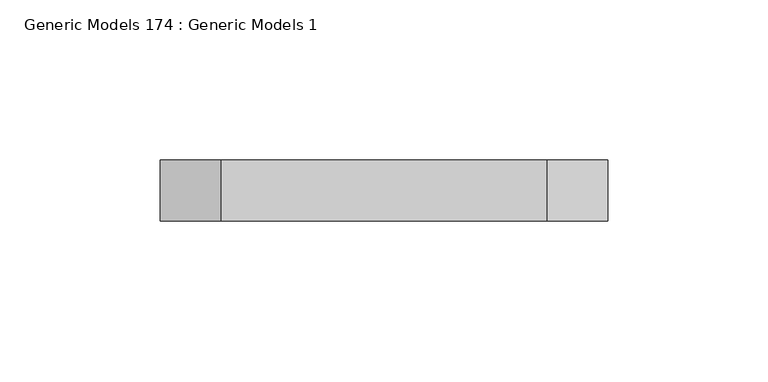
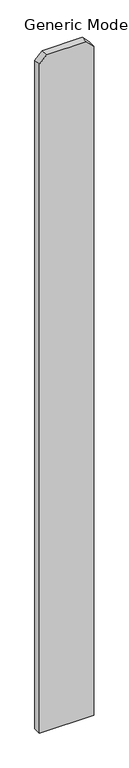
"""IFC4 building model written with IfcOpenShell, lengths in millimetres: proxy geometry, Generic Models 174 : Generic Models 1."""

from ifc_helpers import new_model, si_unit, frame, origin, place, context, project, spatial, polyline, outline, extrude, source, transform, mapped, element, save


def generic_models_174_generic_models_1_c9b0eb3d(model_context):
    return source(origin(), model_context, "Body", "SweptSolid", [
        extrude(outline(polyline([(76.2, 56513.4125), (1885.95, 56513.4125), (1905.0, 56494.3625), (1905.0, 56392.7625), (1885.95, 56373.7125), (76.2, 56373.7125), (76.2, 56513.4125)])), frame((0.0, 547.6875, 0.0), z_axis=(0.0, 1.0, 0.0), x_axis=(0.0, 0.0, 1.0)), (0.0, 0.0, 1.0), 19.05),
    ])


if __name__ == "__main__":
    model = new_model("IFC4")
    model_context = context("Model", 3, world=origin())
    ifc_project = project(units=[si_unit("LENGTHUNIT", "METRE", prefix="MILLI")], contexts=[model_context])
    site = spatial("IfcSite", under=ifc_project)
    building = spatial("IfcBuilding", under=site)
    placement = place(None, origin())
    generic_models_174_generic_models_1_shape = generic_models_174_generic_models_1_c9b0eb3d(model_context)
    element("IfcBuildingElementProxy", 1, Name="Generic Models 174 : Generic Models 1", ObjectType="Generic Models 174 : Generic Models 1", at=placement, inside=building, context=model_context, shape_type="MappedRepresentation", body=[
        mapped(generic_models_174_generic_models_1_shape, transform((0.0, 0.0, 0.0), x_axis=(1.0, 0.0, 0.0), y_axis=(0.0, 1.0, 0.0), z_axis=(0.0, 0.0, 1.0))),
    ])
    save(model, "model.ifc")

# Revit data of these elements
# Element 1 (IfcBuildingElementProxy, "Generic Models 174 : Generic Models 1")
#   Materials on its faces: "VERTICAL 1X6 CEDAR PLANKS W/ CLEAR WOOD SEALER"
# Materials
#   "VERTICAL 1X6 CEDAR PLANKS W/ CLEAR WOOD SEALER": class "Wood", colour RGB 234 198 147, transparency 0, Description = "Pinus Echinata", Cost = 0
